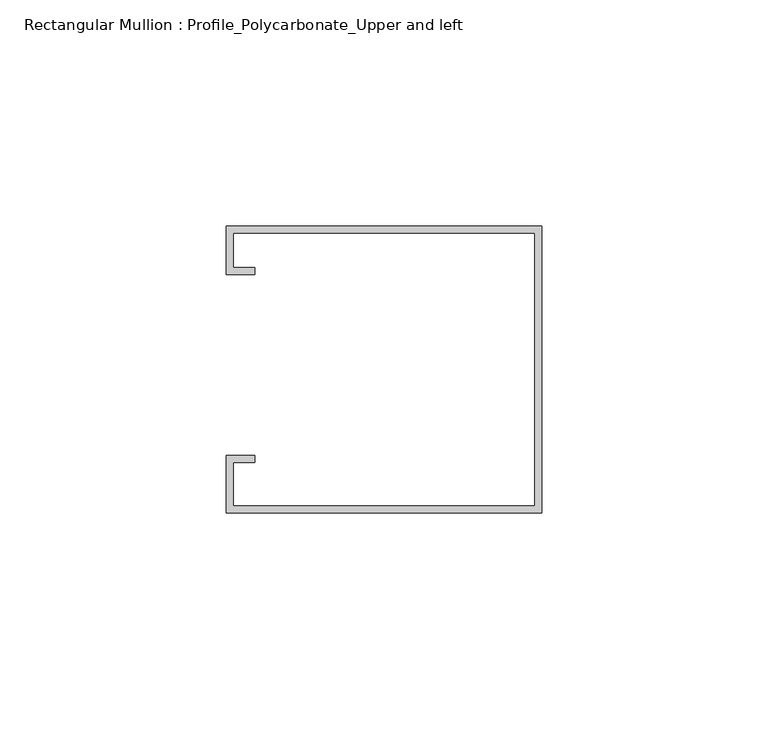
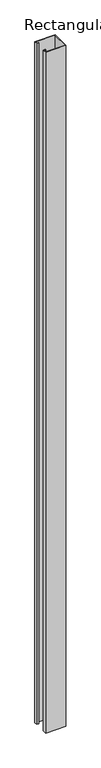
"""IFC4 building model written with IfcOpenShell, lengths in millimetres: member geometry, Rectangular Mullion : Profile_Polycarbonate_Upper and left."""

from ifc_helpers import new_model, si_unit, frame, origin, place, context, project, spatial, polyline, outline, extrude, source, transform, mapped, element, save


def rectangular_mullion_profile_polycarbonate_upper_and_left_5739b8ac(model_context):
    return source(origin(), model_context, "Body", "SweptSolid", [
        extrude(outline(polyline([(0.0, -32.7), (-69.85, -32.7), (-69.85, -20.0), (-63.5, -20.0), (-63.5, -21.5875), (-68.2625, -21.5875), (-68.2625, -31.1125), (-1.5875, -31.1125), (-1.5875, 29.2125), (-68.2625, 29.2125), (-68.2625, 21.5875), (-63.5, 21.5875), (-63.5, 20.0), (-69.85, 20.0), (-69.85, 30.8), (0.0, 30.8), (0.0, -32.7)])), frame((0.0, 0.0, -2479.675), z_axis=(0.0, 0.0, 1.0), x_axis=(1.0, 0.0, 0.0)), (0.0, 0.0, 1.0), 2479.675),
    ])


if __name__ == "__main__":
    model = new_model("IFC4")
    model_context = context("Model", 3, world=origin())
    ifc_project = project(units=[si_unit("LENGTHUNIT", "METRE", prefix="MILLI")], contexts=[model_context])
    site = spatial("IfcSite", under=ifc_project)
    building = spatial("IfcBuilding", under=site)
    placement = place(None, origin())
    rectangular_mullion_profile_polycarbonate_upper_and_left_shape = rectangular_mullion_profile_polycarbonate_upper_and_left_5739b8ac(model_context)
    element("IfcMember", 1, ObjectType="Rectangular Mullion : Profile_Polycarbonate_Upper and left", at=placement, inside=building, context=model_context, shape_type="MappedRepresentation", body=[
        mapped(rectangular_mullion_profile_polycarbonate_upper_and_left_shape, transform((0.0, 0.0, 0.0), x_axis=(1.0, 0.0, 0.0), y_axis=(0.0, 1.0, 0.0), z_axis=(0.0, 0.0, 1.0))),
    ])
    save(model, "model.ifc")

# Revit data of these elements
# Type "Rectangular Mullion : Profile_Polycarbonate_Upper and left"
#   built-in parameter 1007322 = 0.208333 (stored number, unit not read)
#   built-in parameter 1007321 = 0.00520833 (stored number, unit not read)
#   built-in parameter 1007320 = 0 (stored number, unit not read)
# Element 1 (IfcMember, "Rectangular Mullion : Profile_Polycarbonate_Upper and left")
#   Materials on its faces: "ALUMINUM PROFILE AT POLYCARBONATE PANEL"
# Materials
#   "ALUMINUM PROFILE AT POLYCARBONATE PANEL": class "Metal", colour RGB 244 244 244, transparency 0, Description = "Aluminum 6061", Cost = 0
